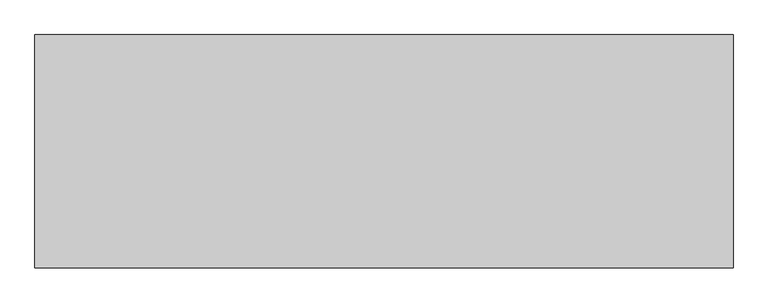
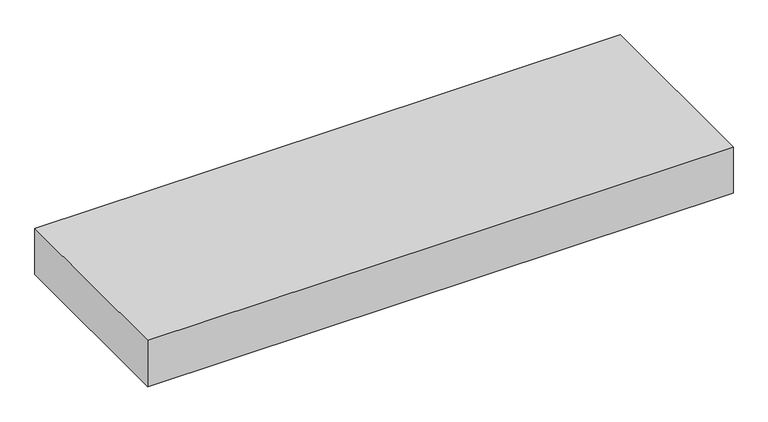
"""IFC4 building model written with IfcOpenShell, lengths in millimetres: furniture geometry, Hearth : Hearth."""

from ifc_helpers import new_model, si_unit, origin, origin_with_axes, place, context, project, spatial, polyline, outline, extrude, source, transform, mapped, element, save


def furniture_4977bb7a(model_context):
    return source(origin(), model_context, "Body", "SweptSolid", [
        extrude(outline(polyline([(1907.591755, 11857.0375), (1907.591755, 11247.4375), (82.55, 11247.4375), (82.55, 11857.0375), (996.95, 11857.0375), (1907.591755, 11857.0375)])), origin_with_axes(), (0.0, 0.0, 1.0), 152.4),
    ])


if __name__ == "__main__":
    model = new_model("IFC4")
    model_context = context("Model", 3, world=origin())
    ifc_project = project(units=[si_unit("LENGTHUNIT", "METRE", prefix="MILLI")], contexts=[model_context])
    site = spatial("IfcSite", under=ifc_project)
    building = spatial("IfcBuilding", under=site)
    placement = place(None, origin())
    furniture_shape = furniture_4977bb7a(model_context)
    element("IfcFurniture", 1, ObjectType="Hearth : Hearth", at=placement, inside=building, context=model_context, shape_type="MappedRepresentation", body=[
        mapped(furniture_shape, transform((0.0, 0.0, 0.0), x_axis=(1.0, 0.0, 0.0), y_axis=(0.0, 1.0, 0.0), z_axis=(0.0, 0.0, 1.0))),
    ])
    save(model, "model.ifc")

# Revit data of these elements
# Type "Hearth : Hearth"
#   COBie.Type = no
# Element 1 (IfcFurniture, "Hearth : Hearth")
#   Materials on its faces: "BoralStone_European-Castle-Stone_Chardonnay-573786"
# Materials
#   "BoralStone_European-Castle-Stone_Chardonnay-573786": class "Stone", colour RGB 137 122 101, transparency 0, Keynote = "04 73 00", Model = "European Castle Stone - Chardonnay 573786", Manufacturer = "Boral Stone Products", URL = "www.culturedstone.com", Description = "Boral Stone Products - European Castle Stone - Chardonnay 573786", C39_Compressive Strength = "1800 psi", Water Absorption = "9%-22%", C482_Shear Bond Strength = "50 psi", Weight = "15 psf", Flame Spread/Smoke Developed = "Flame Spread - 0, Smoke Developed - 0", R Value_Inch = 0.355, Warranty Duration (Years) = 50, MR 5.1 = 1
